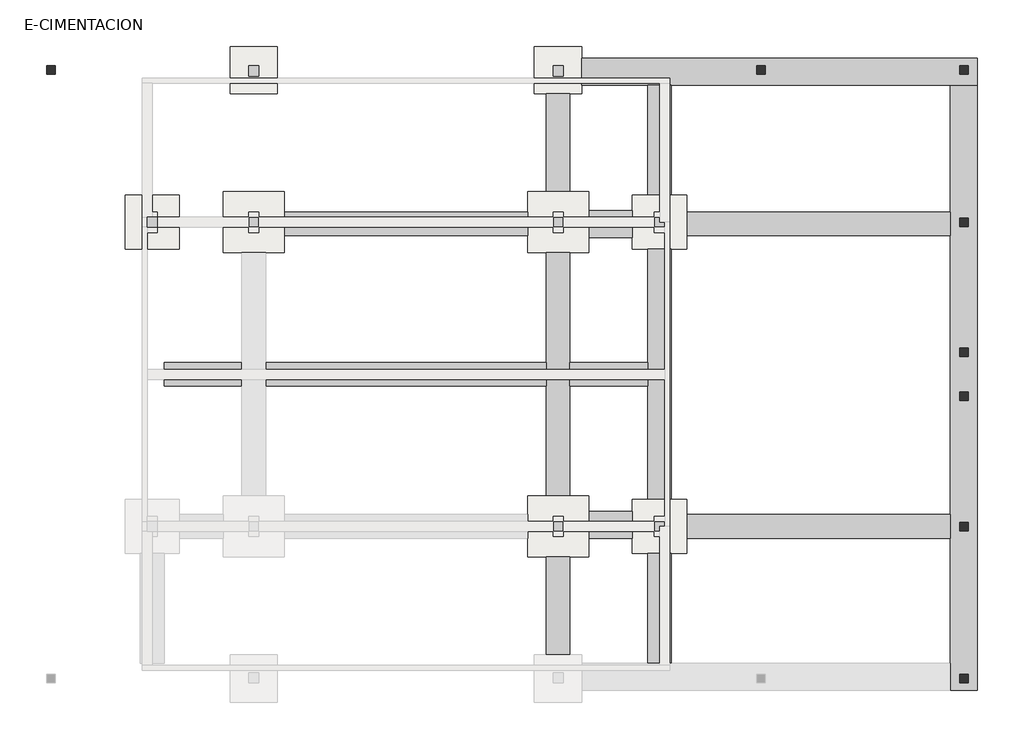
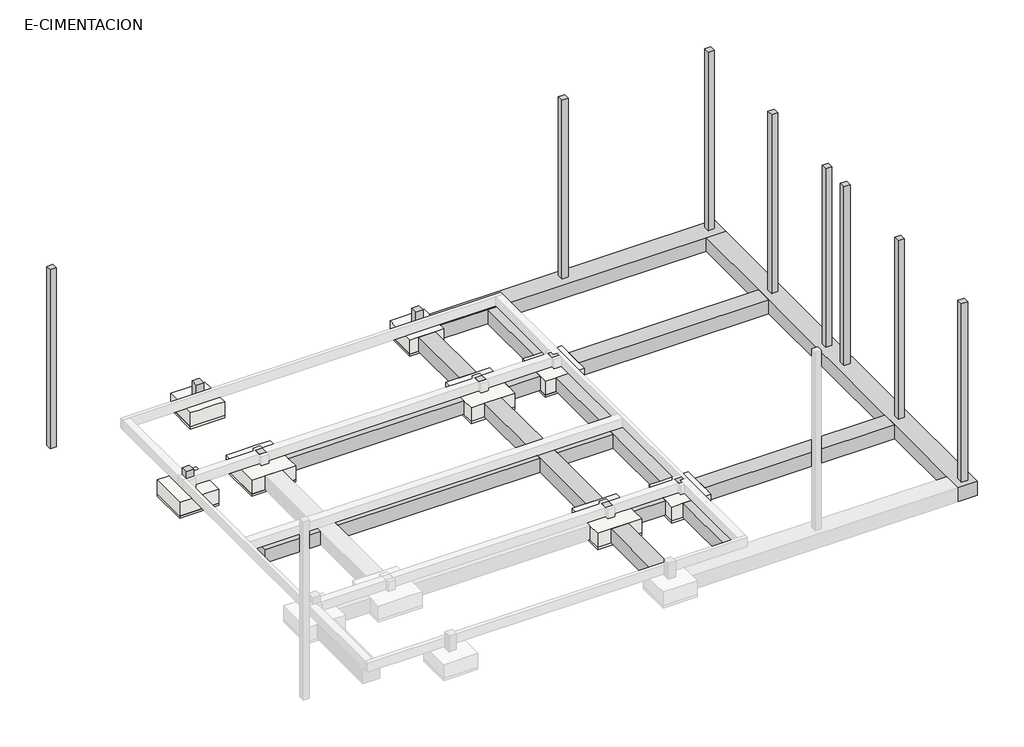
# One storey, part 2 of 2: 16 columns, 14 beams, 8 slabs.
"""IFC4 building model written with IfcOpenShell, lengths in millimetres."""

from ifc_helpers import new_model, si_unit, frame, origin, place, context, project, spatial, polyline, outline, extrude, faceted_brep, element, save

model = new_model("IFC4")

# Units and contexts
model_context = context("Model", 3, world=origin())
ifc_project = project(units=[si_unit("LENGTHUNIT", "METRE", prefix="MILLI")], contexts=[model_context])

# Site, building, storey
site = spatial("IfcSite", under=ifc_project)
building = spatial("IfcBuilding", under=site)
storey = spatial("IfcBuildingStorey", under=building, Name="E-CIMENTACION", Elevation=-900.0)

# Beams
placement = place(None, origin())
element("IfcBeam", 1, ObjectType="E-VIGA-Hormigon : E-VIGA-Hormigon", at=placement, inside=storey, context=model_context, shape_type="SweptSolid", body=[
    extrude(outline(polyline([(-12350.0, -700.0), (-11650.0, -700.0), (-11650.0, -3600.0), (-12350.0, -3600.0), (-12350.0, -700.0)])), frame((0.0, 0.0, -1500.0), z_axis=(0.0, 0.0, 1.0), x_axis=(1.0, 0.0, 0.0)), (0.0, 0.0, 1.0), 600.0),
])
element("IfcBeam", 2, ObjectType="E-VIGA-Hormigon : E-VIGA-Hormigon", at=placement, inside=storey, context=model_context, shape_type="Brep", body=[
    faceted_brep([(-12350.0, -5400.0, -900.0), (-12350.0, -5400.0, -1500.0), (-12350.0, -8650.0, -1500.0), (-12350.0, -9350.0, -1500.0), (-12350.0, -12600.0, -1500.0), (-12350.0, -12600.0, -900.0), (-12350.0, -9350.0, -900.0), (-12350.0, -8650.0, -900.0), (-11650.0, -5400.0, -1500.0), (-11650.0, -8650.0, -1500.0), (-11650.0, -9350.0, -1500.0), (-11650.0, -12600.0, -1500.0), (-11650.0, -5400.0, -900.0), (-11650.0, -8650.0, -900.0), (-11650.0, -9350.0, -900.0), (-11650.0, -12600.0, -900.0)], [[[0, 1, 2, 3, 4, 5, 6, 7]], [[1, 8, 9, 10, 11, 4, 3, 2]], [[8, 12, 13, 14, 15, 11, 10, 9]], [[12, 0, 7, 6, 5, 15, 14, 13]], [[1, 0, 12, 8]], [[5, 4, 11, 15]]]),
])
element("IfcBeam", 3, ObjectType="E-VIGA-Hormigon : E-VIGA-Hormigon", at=placement, inside=storey, context=model_context, shape_type="SweptSolid", body=[
    extrude(outline(polyline([(-11650.0, -17300.0), (-12350.0, -17300.0), (-12350.0, -14400.0), (-11650.0, -14400.0), (-11650.0, -17300.0)])), frame((0.0, 0.0, -1500.0), z_axis=(0.0, 0.0, 1.0), x_axis=(1.0, 0.0, 0.0)), (0.0, 0.0, 1.0), 600.0),
])
element("IfcBeam", 4, ObjectType="E-VIGA-Hormigon : E-VIGA-Hormigon", at=placement, inside=storey, context=model_context, shape_type="Brep", body=[
    faceted_brep([(400.0, -450.0, -1500.0), (400.0, -450.0, -900.0), (-400.0, -450.0, -900.0), (-8650.0, -450.0, -900.0), (-9350.0, -450.0, -900.0), (-11300.0, -450.0, -900.0), (-11300.0, -450.0, -1500.0), (-9350.0, -450.0, -1500.0), (-8650.0, -450.0, -1500.0), (-400.0, -450.0, -1500.0), (400.0, 350.0, -1500.0), (-11300.0, 350.0, -1500.0), (400.0, 350.0, -900.0), (-11300.0, 350.0, -900.0)], [[[0, 1, 2, 3, 4, 5, 6, 7, 8, 9]], [[10, 0, 9, 8, 7, 6, 11]], [[12, 10, 11, 13]], [[1, 12, 13, 5, 4, 3, 2]], [[6, 5, 13, 11]], [[1, 0, 10, 12]]]),
])
element("IfcBeam", 5, ObjectType="E-VIGA-Hormigon : E-VIGA-Hormigon", at=placement, inside=storey, context=model_context, shape_type="Brep", body=[
    faceted_brep([(-400.0, -18350.0, -1500.0), (-400.0, -18350.0, -900.0), (-400.0, -17550.0, -900.0), (-400.0, -13850.0, -900.0), (-400.0, -13150.0, -900.0), (-400.0, -4900.0, -900.0), (-400.0, -4200.0, -900.0), (-400.0, -450.0, -900.0), (-400.0, -450.0, -1500.0), (-400.0, -4200.0, -1500.0), (-400.0, -4900.0, -1500.0), (-400.0, -13150.0, -1500.0), (-400.0, -13850.0, -1500.0), (-400.0, -17550.0, -1500.0), (400.0, -18350.0, -1500.0), (400.0, -450.0, -1500.0), (400.0, -18350.0, -900.0), (400.0, -450.0, -900.0)], [[[0, 1, 2, 3, 4, 5, 6, 7, 8, 9, 10, 11, 12, 13]], [[14, 0, 13, 12, 11, 10, 9, 8, 15]], [[16, 14, 15, 17]], [[1, 16, 17, 7, 6, 5, 4, 3, 2]], [[8, 7, 17, 15]], [[1, 0, 14, 16]]]),
])
element("IfcBeam", 6, ObjectType="E-VIGA-Hormigon : E-VIGA-Hormigon", at=placement, inside=storey, context=model_context, shape_type="SweptSolid", body=[
    extrude(outline(polyline([(-400.0, -4200.0), (-400.0, -4900.0), (-8200.0, -4900.0), (-8200.0, -4200.0), (-400.0, -4200.0)])), frame((0.0, 0.0, -1500.0), z_axis=(0.0, 0.0, 1.0), x_axis=(1.0, 0.0, 0.0)), (0.0, 0.0, 1.0), 600.0),
])
element("IfcBeam", 7, ObjectType="E-VIGA-Hormigon : E-VIGA-Hormigon", at=placement, inside=storey, context=model_context, shape_type="SweptSolid", body=[
    extrude(outline(polyline([(-400.0, -13150.0), (-400.0, -13850.0), (-8200.0, -13850.0), (-8200.0, -13150.0), (-400.0, -13150.0)])), frame((0.0, 0.0, -1500.0), z_axis=(0.0, 0.0, 1.0), x_axis=(1.0, 0.0, 0.0)), (0.0, 0.0, 1.0), 600.0),
])
element("IfcBeam", 8, ObjectType="E-VIGA-Hormigon : E-VIGA-Hormigon", at=placement, inside=storey, context=model_context, shape_type="SweptSolid", body=[
    extrude(outline(polyline([(-11100.0, -4950.0), (-11100.0, -4150.0), (-9800.0, -4150.0), (-9800.0, -4950.0), (-11100.0, -4950.0)])), frame((0.0, 0.0, -1500.0), z_axis=(0.0, 0.0, 1.0), x_axis=(1.0, 0.0, 0.0)), (0.0, 0.0, 1.0), 600.0),
])
element("IfcBeam", 9, ObjectType="E-VIGA-Hormigon : E-VIGA-Hormigon", at=placement, inside=storey, context=model_context, shape_type="SweptSolid", body=[
    extrude(outline(polyline([(-11100.0, -13850.0), (-11100.0, -13050.0), (-9800.0, -13050.0), (-9800.0, -13850.0), (-11100.0, -13850.0)])), frame((0.0, 0.0, -1500.0), z_axis=(0.0, 0.0, 1.0), x_axis=(1.0, 0.0, 0.0)), (0.0, 0.0, 1.0), 600.0),
])
element("IfcBeam", 10, ObjectType="E-VIGA-Hormigon : E-VIGA-Hormigon", at=placement, inside=storey, context=model_context, shape_type="SweptSolid", body=[
    extrude(outline(polyline([(-20100.0, -4900.0), (-20100.0, -4200.0), (-12900.0, -4200.0), (-12900.0, -4900.0), (-20100.0, -4900.0)])), frame((0.0, 0.0, -1500.0), z_axis=(0.0, 0.0, 1.0), x_axis=(1.0, 0.0, 0.0)), (0.0, 0.0, 1.0), 600.0),
])
element("IfcBeam", 11, ObjectType="E-VIGA-Hormigon : E-VIGA-Hormigon", at=placement, inside=storey, context=model_context, shape_type="Brep", body=[
    faceted_brep([(-9350.0, -5300.0, -900.0), (-9350.0, -5300.0, -1500.0), (-9350.0, -8650.0, -1500.0), (-9350.0, -9350.0, -1500.0), (-9350.0, -12700.0, -1500.0), (-9350.0, -12700.0, -900.0), (-9350.0, -9350.0, -900.0), (-9350.0, -8650.0, -900.0), (-8650.0, -5300.0, -1500.0), (-8650.0, -12700.0, -1500.0), (-8650.0, -5300.0, -900.0), (-8650.0, -12700.0, -900.0)], [[[0, 1, 2, 3, 4, 5, 6, 7]], [[1, 8, 9, 4, 3, 2]], [[8, 10, 11, 9]], [[10, 0, 7, 6, 5, 11]], [[1, 0, 10, 8]], [[5, 4, 9, 11]]]),
])
element("IfcBeam", 12, ObjectType="E-VIGA-Hormigon : E-VIGA-Hormigon", at=placement, inside=storey, context=model_context, shape_type="SweptSolid", body=[
    extrude(outline(polyline([(-9350.0, -450.0), (-8650.0, -450.0), (-8650.0, -3700.0), (-9350.0, -3700.0), (-9350.0, -450.0)])), frame((0.0, 0.0, -1500.0), z_axis=(0.0, 0.0, 1.0), x_axis=(1.0, 0.0, 0.0)), (0.0, 0.0, 1.0), 600.0),
])
element("IfcBeam", 13, ObjectType="E-VIGA-Hormigon : E-VIGA-Hormigon", at=placement, inside=storey, context=model_context, shape_type="SweptSolid", body=[
    extrude(outline(polyline([(-8650.0, -17550.0), (-9350.0, -17550.0), (-9350.0, -14300.0), (-8650.0, -14300.0), (-8650.0, -17550.0)])), frame((0.0, 0.0, -1500.0), z_axis=(0.0, 0.0, 1.0), x_axis=(1.0, 0.0, 0.0)), (0.0, 0.0, 1.0), 600.0),
])
element("IfcBeam", 14, ObjectType="E-VIGA-Hormigon : E-VIGA-Hormigon", at=placement, inside=storey, context=model_context, shape_type="SweptSolid", body=[
    extrude(outline(polyline([(-9350.0, -8650.0), (-9350.0, -9350.0), (-11650.0, -9350.0), (-11650.0, -8650.0), (-9350.0, -8650.0)])), frame((0.0, 0.0, -1500.0), z_axis=(0.0, 0.0, 1.0), x_axis=(1.0, 0.0, 0.0)), (0.0, 0.0, 1.0), 600.0),
    extrude(outline(polyline([(-23650.0, -9350.0), (-23650.0, -8650.0), (-21350.0, -8650.0), (-21350.0, -9350.0), (-23650.0, -9350.0)])), frame((0.0, 0.0, -1500.0), z_axis=(0.0, 0.0, 1.0), x_axis=(1.0, 0.0, 0.0)), (0.0, 0.0, 1.0), 600.0),
    extrude(outline(polyline([(-12350.0, -8650.0), (-12350.0, -9350.0), (-20650.0, -9350.0), (-20650.0, -8650.0), (-12350.0, -8650.0)])), frame((0.0, 0.0, -1500.0), z_axis=(0.0, 0.0, 1.0), x_axis=(1.0, 0.0, 0.0)), (0.0, 0.0, 1.0), 600.0),
])

# Columns
element("IfcColumn", 15, ObjectType="Hormigón-Cuadrado-Pilar : PILAR 25X25", at=placement, inside=storey, context=model_context, shape_type="SweptSolid", body=[
    extrude(outline(polyline([(-26875.0, 125.0), (-26875.0, -125.0), (-27125.0, -125.0), (-27125.0, 125.0), (-26875.0, 125.0)])), frame((0.0, 0.0, -900.0), z_axis=(0.0, 0.0, 1.0), x_axis=(1.0, 0.0, 0.0)), (0.0, 0.0, 1.0), 7750.0),
])
element("IfcColumn", 16, ObjectType="Hormigón-Cuadrado-Pilar : PILAR 25X25", at=placement, inside=storey, context=model_context, shape_type="SweptSolid", body=[
    extrude(outline(polyline([(125.0, 125.0), (125.0, -125.0), (-125.0, -125.0), (-125.0, 125.0), (125.0, 125.0)])), frame((0.0, 0.0, -900.0), z_axis=(0.0, 0.0, 1.0), x_axis=(1.0, 0.0, 0.0)), (0.0, 0.0, 1.0), 7750.0),
])
element("IfcColumn", 17, ObjectType="Hormigón-Cuadrado-Pilar : PILAR 25X25", at=placement, inside=storey, context=model_context, shape_type="SweptSolid", body=[
    extrude(outline(polyline([(125.0, -4375.0), (125.0, -4625.0), (-125.0, -4625.0), (-125.0, -4375.0), (125.0, -4375.0)])), frame((0.0, 0.0, -900.0), z_axis=(0.0, 0.0, 1.0), x_axis=(1.0, 0.0, 0.0)), (0.0, 0.0, 1.0), 7750.0),
])
element("IfcColumn", 18, ObjectType="Hormigón-Cuadrado-Pilar : PILAR 25X25", at=placement, inside=storey, context=model_context, shape_type="Brep", body=[
    faceted_brep([(125.0, -8225.0, -900.0), (125.0, -8475.0, -900.0), (-125.0, -8475.0, -900.0), (-125.0, -8225.0, -900.0), (125.0, -8225.0, 6850.0), (125.0, -8475.0, 6850.0), (125.0, -8225.0, 2480.0), (125.0, -8225.0, 2730.0), (125.0, -8225.0, 6600.0), (-125.0, -8475.0, 6850.0), (-125.0, -8225.0, 6850.0), (-125.0, -8225.0, 6600.0), (-125.0, -8225.0, 2730.0), (-125.0, -8225.0, 2480.0)], [[[0, 1, 2, 3]], [[4, 5, 1, 0, 6, 7, 8]], [[5, 9, 2, 1]], [[9, 10, 11, 12, 13, 3, 2]], [[10, 4, 8, 7, 6, 0, 3, 13, 12, 11]], [[4, 10, 9, 5]]]),
])
element("IfcColumn", 19, ObjectType="Hormigón-Cuadrado-Pilar : PILAR 25X25", at=placement, inside=storey, context=model_context, shape_type="SweptSolid", body=[
    extrude(outline(polyline([(125.0, -13375.0), (125.0, -13625.0), (-125.0, -13625.0), (-125.0, -13375.0), (125.0, -13375.0)])), frame((0.0, 0.0, -900.0), z_axis=(0.0, 0.0, 1.0), x_axis=(1.0, 0.0, 0.0)), (0.0, 0.0, 1.0), 7750.0),
])
element("IfcColumn", 20, ObjectType="Hormigón-Cuadrado-Pilar : PILAR 25X25", at=placement, inside=storey, context=model_context, shape_type="SweptSolid", body=[
    extrude(outline(polyline([(125.0, -17875.0), (125.0, -18125.0), (-125.0, -18125.0), (-125.0, -17875.0), (125.0, -17875.0)])), frame((0.0, 0.0, -900.0), z_axis=(0.0, 0.0, 1.0), x_axis=(1.0, 0.0, 0.0)), (0.0, 0.0, 1.0), 7750.0),
])
element("IfcColumn", 21, ObjectType="Hormigón-Cuadrado-Pilar : PILAR 25X25", at=placement, inside=storey, context=model_context, shape_type="SweptSolid", body=[
    extrude(outline(polyline([(-5875.0, 125.0), (-5875.0, -125.0), (-6125.0, -125.0), (-6125.0, 125.0), (-5875.0, 125.0)])), frame((0.0, 0.0, -900.0), z_axis=(0.0, 0.0, 1.0), x_axis=(1.0, 0.0, 0.0)), (0.0, 0.0, 1.0), 7750.0),
])
element("IfcColumn", 22, ObjectType="Hormigón-Cuadrado-Pilar : PILAR 25X25", at=placement, inside=storey, context=model_context, shape_type="Brep", body=[
    faceted_brep([(125.0, -9775.0, -900.0), (-125.0, -9775.0, -900.0), (-125.0, -9525.0, -900.0), (125.0, -9525.0, -900.0), (125.0, -9775.0, 6850.0), (125.0, -9775.0, 6600.0), (125.0, -9775.0, 2730.0), (125.0, -9775.0, 2480.0), (125.0, -9525.0, 6850.0), (-125.0, -9525.0, 6850.0), (-125.0, -9775.0, 2480.0), (-125.0, -9775.0, 2730.0), (-125.0, -9775.0, 6600.0), (-125.0, -9775.0, 6850.0)], [[[0, 1, 2, 3]], [[4, 5, 6, 7, 0, 3, 8]], [[8, 3, 2, 9]], [[9, 2, 1, 10, 11, 12, 13]], [[13, 12, 11, 10, 1, 0, 7, 6, 5, 4]], [[4, 8, 9, 13]]]),
])
element("IfcColumn", 23, ObjectType="Hormigón-Cuadrado-Pilar : PILAR 30X30", at=placement, inside=storey, context=model_context, shape_type="SweptSolid", body=[
    extrude(outline(polyline([(-20850.0, 125.0), (-20850.0, -175.0), (-21150.0, -175.0), (-21150.0, 125.0), (-20850.0, 125.0)])), frame((0.0, 0.0, -900.0), z_axis=(0.0, 0.0, 1.0), x_axis=(1.0, 0.0, 0.0)), (0.0, 0.0, 1.0), 700.0),
])
element("IfcColumn", 24, ObjectType="Hormigón-Cuadrado-Pilar : PILAR 30X30", at=placement, inside=storey, context=model_context, shape_type="SweptSolid", body=[
    extrude(outline(polyline([(-11850.0, 125.0), (-11850.0, -175.0), (-12150.0, -175.0), (-12150.0, 125.0), (-11850.0, 125.0)])), frame((0.0, 0.0, -900.0), z_axis=(0.0, 0.0, 1.0), x_axis=(1.0, 0.0, 0.0)), (0.0, 0.0, 1.0), 700.0),
])
element("IfcColumn", 25, ObjectType="Hormigón-Cuadrado-Pilar : PILAR 30X30", at=placement, inside=storey, context=model_context, shape_type="SweptSolid", body=[
    extrude(outline(polyline([(-20850.0, -4350.0), (-20850.0, -4650.0), (-21150.0, -4650.0), (-21150.0, -4350.0), (-20850.0, -4350.0)])), frame((0.0, 0.0, -900.0), z_axis=(0.0, 0.0, 1.0), x_axis=(1.0, 0.0, 0.0)), (0.0, 0.0, 1.0), 400.0),
])
element("IfcColumn", 26, ObjectType="Hormigón-Cuadrado-Pilar : PILAR 30X30", at=placement, inside=storey, context=model_context, shape_type="SweptSolid", body=[
    extrude(outline(polyline([(-11850.0, -13350.0), (-11850.0, -13650.0), (-12150.0, -13650.0), (-12150.0, -13350.0), (-11850.0, -13350.0)])), frame((0.0, 0.0, -900.0), z_axis=(0.0, 0.0, 1.0), x_axis=(1.0, 0.0, 0.0)), (0.0, 0.0, 1.0), 400.0),
])
element("IfcColumn", 27, ObjectType="Hormigón-Cuadrado-Pilar : PILAR 30X30", at=placement, inside=storey, context=model_context, shape_type="SweptSolid", body=[
    extrude(outline(polyline([(-11850.0, -4350.0), (-11850.0, -4650.0), (-12150.0, -4650.0), (-12150.0, -4350.0), (-11850.0, -4350.0)])), frame((0.0, 0.0, -900.0), z_axis=(0.0, 0.0, 1.0), x_axis=(1.0, 0.0, 0.0)), (0.0, 0.0, 1.0), 400.0),
])
element("IfcColumn", 28, ObjectType="Hormigón-Cuadrado-Pilar : PILAR 30X30", at=placement, inside=storey, context=model_context, shape_type="SweptSolid", body=[
    extrude(outline(polyline([(-23850.0, -4350.0), (-23850.0, -4650.0), (-24150.0, -4650.0), (-24150.0, -4350.0), (-23850.0, -4350.0)])), frame((0.0, 0.0, -500.0), z_axis=(0.0, 0.0, 1.0), x_axis=(1.0, 0.0, 0.0)), (0.0, 0.0, 1.0), 300.0),
])
element("IfcColumn", 29, ObjectType="Hormigón-Cuadrado-Pilar : PILAR 30X30", at=placement, inside=storey, context=model_context, shape_type="SweptSolid", body=[
    extrude(outline(polyline([(-9150.0, -13650.0), (-9150.0, -13350.0), (-8850.0, -13350.0), (-8850.0, -13500.0), (-9000.0, -13500.0), (-9000.0, -13650.0), (-9150.0, -13650.0)])), frame((0.0, 0.0, -900.0), z_axis=(0.0, 0.0, 1.0), x_axis=(1.0, 0.0, 0.0)), (0.0, 0.0, 1.0), 400.0),
])
element("IfcColumn", 30, ObjectType="Hormigón-Cuadrado-Pilar : PILAR 30X30", at=placement, inside=storey, context=model_context, shape_type="SweptSolid", body=[
    extrude(outline(polyline([(-8850.0, -4650.0), (-9150.0, -4650.0), (-9150.0, -4350.0), (-9000.0, -4350.0), (-9000.0, -4500.0), (-8850.0, -4500.0), (-8850.0, -4650.0)])), frame((0.0, 0.0, -900.0), z_axis=(0.0, 0.0, 1.0), x_axis=(1.0, 0.0, 0.0)), (0.0, 0.0, 1.0), 400.0),
])

# Slabs
element("IfcSlab", 31, ObjectType="E-ZAPATA : E-ZAPATA", at=placement, inside=storey, context=model_context, shape_type="SolidModel", body=[
    faceted_brep([(-12700.0, 700.0, -900.0), (-12700.0, 350.0, -900.0), (-12700.0, -450.0, -900.0), (-12700.0, -700.0, -900.0), (-12350.0, -700.0, -900.0), (-11650.0, -700.0, -900.0), (-11300.0, -700.0, -900.0), (-11300.0, -450.0, -900.0), (-11300.0, 350.0, -900.0), (-11300.0, 700.0, -900.0), (-12700.0, 700.0, -1500.0), (-11300.0, 700.0, -1500.0), (-11300.0, 350.0, -1500.0), (-11300.0, -450.0, -1500.0), (-11300.0, -700.0, -1500.0), (-11650.0, -700.0, -1500.0), (-12350.0, -700.0, -1500.0), (-12700.0, -700.0, -1500.0), (-12700.0, -450.0, -1500.0), (-12700.0, 350.0, -1500.0)], [[[0, 1, 2, 3, 4, 5, 6, 7, 8, 9]], [[10, 11, 12, 13, 14, 15, 16, 17, 18, 19]], [[0, 9, 11, 10]], [[9, 8, 7, 6, 14, 13, 12, 11]], [[6, 5, 4, 3, 17, 16, 15, 14]], [[3, 2, 1, 0, 10, 19, 18, 17]]]),
    extrude(outline(polyline([(-11300.0, 700.0), (-11300.0, -700.0), (-12700.0, -700.0), (-12700.0, 700.0), (-11300.0, 700.0)])), frame((0.0, 0.0, -1600.0), z_axis=(0.0, 0.0, 1.0), x_axis=(1.0, 0.0, 0.0)), (0.0, 0.0, 1.0), 100.0),
])
element("IfcSlab", 32, ObjectType="E-ZAPATA : E-ZAPATA", at=placement, inside=storey, context=model_context, shape_type="SolidModel", body=[
    faceted_brep([(-21900.0, -3600.0, -900.0), (-21900.0, -4150.0, -900.0), (-21900.0, -4950.0, -900.0), (-21900.0, -5400.0, -900.0), (-21350.0, -5400.0, -900.0), (-20650.0, -5400.0, -900.0), (-20100.0, -5400.0, -900.0), (-20100.0, -4900.0, -900.0), (-20100.0, -4200.0, -900.0), (-20100.0, -3600.0, -900.0), (-20650.0, -3600.0, -900.0), (-21350.0, -3600.0, -900.0), (-21900.0, -3600.0, -1500.0), (-21350.0, -3600.0, -1500.0), (-20650.0, -3600.0, -1500.0), (-20100.0, -3600.0, -1500.0), (-20100.0, -4200.0, -1500.0), (-20100.0, -4900.0, -1500.0), (-20100.0, -5400.0, -1500.0), (-20650.0, -5400.0, -1500.0), (-21350.0, -5400.0, -1500.0), (-21900.0, -5400.0, -1500.0), (-21900.0, -4950.0, -1500.0), (-21900.0, -4150.0, -1500.0)], [[[0, 1, 2, 3, 4, 5, 6, 7, 8, 9, 10, 11]], [[12, 13, 14, 15, 16, 17, 18, 19, 20, 21, 22, 23]], [[0, 11, 10, 9, 15, 14, 13, 12]], [[9, 8, 7, 6, 18, 17, 16, 15]], [[6, 5, 4, 3, 21, 20, 19, 18]], [[3, 2, 1, 0, 12, 23, 22, 21]]]),
    extrude(outline(polyline([(-20100.0, -3600.0), (-20100.0, -5400.0), (-21900.0, -5400.0), (-21900.0, -3600.0), (-20100.0, -3600.0)])), frame((0.0, 0.0, -1600.0), z_axis=(0.0, 0.0, 1.0), x_axis=(1.0, 0.0, 0.0)), (0.0, 0.0, 1.0), 100.0),
])
element("IfcSlab", 33, ObjectType="E-ZAPATA : E-ZAPATA", at=placement, inside=storey, context=model_context, shape_type="SolidModel", body=[
    faceted_brep([(-12900.0, -3600.0, -900.0), (-12900.0, -4200.0, -900.0), (-12900.0, -4900.0, -900.0), (-12900.0, -5400.0, -900.0), (-12350.0, -5400.0, -900.0), (-11650.0, -5400.0, -900.0), (-11100.0, -5400.0, -900.0), (-11100.0, -4950.0, -900.0), (-11100.0, -4150.0, -900.0), (-11100.0, -3600.0, -900.0), (-11650.0, -3600.0, -900.0), (-12350.0, -3600.0, -900.0), (-12900.0, -3600.0, -1500.0), (-12350.0, -3600.0, -1500.0), (-11650.0, -3600.0, -1500.0), (-11100.0, -3600.0, -1500.0), (-11100.0, -4150.0, -1500.0), (-11100.0, -4950.0, -1500.0), (-11100.0, -5400.0, -1500.0), (-11650.0, -5400.0, -1500.0), (-12350.0, -5400.0, -1500.0), (-12900.0, -5400.0, -1500.0), (-12900.0, -4900.0, -1500.0), (-12900.0, -4200.0, -1500.0)], [[[0, 1, 2, 3, 4, 5, 6, 7, 8, 9, 10, 11]], [[12, 13, 14, 15, 16, 17, 18, 19, 20, 21, 22, 23]], [[0, 11, 10, 9, 15, 14, 13, 12]], [[9, 8, 7, 6, 18, 17, 16, 15]], [[6, 5, 4, 3, 21, 20, 19, 18]], [[3, 2, 1, 0, 12, 23, 22, 21]]]),
    extrude(outline(polyline([(-11100.0, -3600.0), (-11100.0, -5400.0), (-12900.0, -5400.0), (-12900.0, -3600.0), (-11100.0, -3600.0)])), frame((0.0, 0.0, -1600.0), z_axis=(0.0, 0.0, 1.0), x_axis=(1.0, 0.0, 0.0)), (0.0, 0.0, 1.0), 100.0),
])
element("IfcSlab", 34, ObjectType="E-ZAPATA : E-ZAPATA", at=placement, inside=storey, context=model_context, shape_type="SolidModel", body=[
    faceted_brep([(-24800.0, -5300.0, -900.0), (-24350.0, -5300.0, -900.0), (-23650.0, -5300.0, -900.0), (-23200.0, -5300.0, -900.0), (-23200.0, -4950.0, -900.0), (-23200.0, -4150.0, -900.0), (-23200.0, -3700.0, -900.0), (-23650.0, -3700.0, -900.0), (-24350.0, -3700.0, -900.0), (-24800.0, -3700.0, -900.0), (-24800.0, -5300.0, -1500.0), (-24800.0, -3700.0, -1500.0), (-24350.0, -3700.0, -1500.0), (-23650.0, -3700.0, -1500.0), (-23200.0, -3700.0, -1500.0), (-23200.0, -4150.0, -1500.0), (-23200.0, -4950.0, -1500.0), (-23200.0, -5300.0, -1500.0), (-23650.0, -5300.0, -1500.0), (-24350.0, -5300.0, -1500.0)], [[[0, 1, 2, 3, 4, 5, 6, 7, 8, 9]], [[10, 11, 12, 13, 14, 15, 16, 17, 18, 19]], [[0, 9, 11, 10]], [[9, 8, 7, 6, 14, 13, 12, 11]], [[6, 5, 4, 3, 17, 16, 15, 14]], [[3, 2, 1, 0, 10, 19, 18, 17]]]),
    extrude(outline(polyline([(-24800.0, -3700.0), (-23200.0, -3700.0), (-23200.0, -5300.0), (-24800.0, -5300.0), (-24800.0, -3700.0)])), frame((0.0, 0.0, -1600.0), z_axis=(0.0, 0.0, 1.0), x_axis=(1.0, 0.0, 0.0)), (0.0, 0.0, 1.0), 100.0),
])
element("IfcSlab", 35, ObjectType="E-ZAPATA : E-ZAPATA", at=placement, inside=storey, context=model_context, shape_type="SolidModel", body=[
    faceted_brep([(-9800.0, -3700.0, -900.0), (-9800.0, -4150.0, -900.0), (-9800.0, -4950.0, -900.0), (-9800.0, -5300.0, -900.0), (-9350.0, -5300.0, -900.0), (-8650.0, -5300.0, -900.0), (-8200.0, -5300.0, -900.0), (-8200.0, -4900.0, -900.0), (-8200.0, -4200.0, -900.0), (-8200.0, -3700.0, -900.0), (-8650.0, -3700.0, -900.0), (-9350.0, -3700.0, -900.0), (-9800.0, -3700.0, -1500.0), (-9350.0, -3700.0, -1500.0), (-8650.0, -3700.0, -1500.0), (-8200.0, -3700.0, -1500.0), (-8200.0, -4200.0, -1500.0), (-8200.0, -4900.0, -1500.0), (-8200.0, -5300.0, -1500.0), (-8650.0, -5300.0, -1500.0), (-9350.0, -5300.0, -1500.0), (-9800.0, -5300.0, -1500.0), (-9800.0, -4950.0, -1500.0), (-9800.0, -4150.0, -1500.0)], [[[0, 1, 2, 3, 4, 5, 6, 7, 8, 9, 10, 11]], [[12, 13, 14, 15, 16, 17, 18, 19, 20, 21, 22, 23]], [[0, 11, 10, 9, 15, 14, 13, 12]], [[9, 8, 7, 6, 18, 17, 16, 15]], [[6, 5, 4, 3, 21, 20, 19, 18]], [[3, 2, 1, 0, 12, 23, 22, 21]]]),
    extrude(outline(polyline([(-8200.0, -3700.0), (-8200.0, -5300.0), (-9800.0, -5300.0), (-9800.0, -3700.0), (-8200.0, -3700.0)])), frame((0.0, 0.0, -1600.0), z_axis=(0.0, 0.0, 1.0), x_axis=(1.0, 0.0, 0.0)), (0.0, 0.0, 1.0), 100.0),
])
element("IfcSlab", 36, ObjectType="E-ZAPATA : E-ZAPATA", at=placement, inside=storey, context=model_context, shape_type="SolidModel", body=[
    faceted_brep([(-12900.0, -14400.0, -900.0), (-12350.0, -14400.0, -900.0), (-11650.0, -14400.0, -900.0), (-11100.0, -14400.0, -900.0), (-11100.0, -13850.0, -900.0), (-11100.0, -13050.0, -900.0), (-11100.0, -12600.0, -900.0), (-11650.0, -12600.0, -900.0), (-12350.0, -12600.0, -900.0), (-12900.0, -12600.0, -900.0), (-12900.0, -13150.0, -900.0), (-12900.0, -13850.0, -900.0), (-12900.0, -14400.0, -1500.0), (-12900.0, -13850.0, -1500.0), (-12900.0, -13150.0, -1500.0), (-12900.0, -12600.0, -1500.0), (-12350.0, -12600.0, -1500.0), (-11650.0, -12600.0, -1500.0), (-11100.0, -12600.0, -1500.0), (-11100.0, -13050.0, -1500.0), (-11100.0, -13850.0, -1500.0), (-11100.0, -14400.0, -1500.0), (-11650.0, -14400.0, -1500.0), (-12350.0, -14400.0, -1500.0)], [[[0, 1, 2, 3, 4, 5, 6, 7, 8, 9, 10, 11]], [[12, 13, 14, 15, 16, 17, 18, 19, 20, 21, 22, 23]], [[0, 12, 23, 22, 21, 3, 2, 1]], [[3, 21, 20, 19, 18, 6, 5, 4]], [[6, 18, 17, 16, 15, 9, 8, 7]], [[9, 15, 14, 13, 12, 0, 11, 10]]]),
    extrude(outline(polyline([(-11100.0, -14400.0), (-12900.0, -14400.0), (-12900.0, -12600.0), (-11100.0, -12600.0), (-11100.0, -14400.0)])), frame((0.0, 0.0, -1600.0), z_axis=(0.0, 0.0, 1.0), x_axis=(1.0, 0.0, 0.0)), (0.0, 0.0, 1.0), 100.0),
])
element("IfcSlab", 37, ObjectType="E-ZAPATA : E-ZAPATA", at=placement, inside=storey, context=model_context, shape_type="SolidModel", body=[
    faceted_brep([(-9800.0, -14300.0, -900.0), (-9350.0, -14300.0, -900.0), (-8650.0, -14300.0, -900.0), (-8200.0, -14300.0, -900.0), (-8200.0, -13850.0, -900.0), (-8200.0, -13150.0, -900.0), (-8200.0, -12700.0, -900.0), (-8650.0, -12700.0, -900.0), (-9350.0, -12700.0, -900.0), (-9800.0, -12700.0, -900.0), (-9800.0, -13050.0, -900.0), (-9800.0, -13850.0, -900.0), (-9800.0, -14300.0, -1500.0), (-9800.0, -13850.0, -1500.0), (-9800.0, -13050.0, -1500.0), (-9800.0, -12700.0, -1500.0), (-9350.0, -12700.0, -1500.0), (-8650.0, -12700.0, -1500.0), (-8200.0, -12700.0, -1500.0), (-8200.0, -13150.0, -1500.0), (-8200.0, -13850.0, -1500.0), (-8200.0, -14300.0, -1500.0), (-8650.0, -14300.0, -1500.0), (-9350.0, -14300.0, -1500.0)], [[[0, 1, 2, 3, 4, 5, 6, 7, 8, 9, 10, 11]], [[12, 13, 14, 15, 16, 17, 18, 19, 20, 21, 22, 23]], [[0, 12, 23, 22, 21, 3, 2, 1]], [[3, 21, 20, 19, 18, 6, 5, 4]], [[6, 18, 17, 16, 15, 9, 8, 7]], [[9, 15, 14, 13, 12, 0, 11, 10]]]),
    extrude(outline(polyline([(-8200.0, -14300.0), (-9800.0, -14300.0), (-9800.0, -12700.0), (-8200.0, -12700.0), (-8200.0, -14300.0)])), frame((0.0, 0.0, -1600.0), z_axis=(0.0, 0.0, 1.0), x_axis=(1.0, 0.0, 0.0)), (0.0, 0.0, 1.0), 100.0),
])
element("IfcSlab", 38, ObjectType="E-ZAPATA : E-ZAPATA", at=placement, inside=storey, context=model_context, shape_type="SolidModel", body=[
    faceted_brep([(-21700.0, 700.0, -900.0), (-21700.0, 350.0, -900.0), (-21700.0, -450.0, -900.0), (-21700.0, -700.0, -900.0), (-21350.0, -700.0, -900.0), (-20650.0, -700.0, -900.0), (-20300.0, -700.0, -900.0), (-20300.0, -450.0, -900.0), (-20300.0, 350.0, -900.0), (-20300.0, 700.0, -900.0), (-21700.0, 700.0, -1500.0), (-20300.0, 700.0, -1500.0), (-20300.0, 350.0, -1500.0), (-20300.0, -450.0, -1500.0), (-20300.0, -700.0, -1500.0), (-20650.0, -700.0, -1500.0), (-21350.0, -700.0, -1500.0), (-21700.0, -700.0, -1500.0), (-21700.0, -450.0, -1500.0), (-21700.0, 350.0, -1500.0)], [[[0, 1, 2, 3, 4, 5, 6, 7, 8, 9]], [[10, 11, 12, 13, 14, 15, 16, 17, 18, 19]], [[0, 9, 11, 10]], [[9, 8, 7, 6, 14, 13, 12, 11]], [[6, 5, 4, 3, 17, 16, 15, 14]], [[3, 2, 1, 0, 10, 19, 18, 17]]]),
    extrude(outline(polyline([(-20300.0, 700.0), (-20300.0, -700.0), (-21700.0, -700.0), (-21700.0, 700.0), (-20300.0, 700.0)])), frame((0.0, 0.0, -1600.0), z_axis=(0.0, 0.0, 1.0), x_axis=(1.0, 0.0, 0.0)), (0.0, 0.0, 1.0), 100.0),
])

save(model, "model.ifc")

# Revit data of these elements
# Type "E-VIGA-Hormigon : E-VIGA-Hormigon"
#   Numeration [instance default] = ""
#   Length [instance default] = 3.000 m
#   AnchoViga [instance default] = 0.200 m
#   AltoViga [instance default] = 0.300 m
# Type "Hormigón-Cuadrado-Pilar : PILAR 25X25"
#   b = 0.250 m
#   Structural Material [instance default] = Hormigón - Hormigón moldeado in situ
# Type "Hormigón-Cuadrado-Pilar : PILAR 30X30"
#   b = 0.300 m
#   Structural Material [instance default] = Hormigón - Hormigón moldeado in situ
# Type "E-ZAPATA : E-ZAPATA"
#   y1 [instance default] = 0.500 m
#   x1 [instance default] = 0.500 m
#   GrosorHormigonLimpieza [instance default] = 0.100 m
#   Width [instance default] = 1.000 m
#   Length [instance default] = 1.000 m
#   Foundation Thickness [instance default] = 0.500 m
#   ColocacionEjeY [instance default] = no
#   ColocacionEjeX [instance default] = no
#   HormigonLimpieza = none
#   Structural Material = none
# Elements 1, 2, 3, 6, 7, 10, 11, 12, 13, 14 (IfcBeam, "E-VIGA-Hormigon : E-VIGA-Hormigon")
#   Comments = ""
#   Numeration = ""
#   AnchoViga = 0.700 m
#   AltoViga = 0.600 m
#   Phase Created = Nueva construcción
#   Materials on its faces: "Concrete, Cast-in-Place, Gray"
# Elements 4, 5, 9 (IfcBeam, "E-VIGA-Hormigon : E-VIGA-Hormigon")
#   Comments = ""
#   Numeration = ""
#   AnchoViga = 0.800 m
#   AltoViga = 0.600 m
#   Phase Created = Nueva construcción
#   Materials on its faces: "Concrete, Cast-in-Place, Gray"
# Element 8 (IfcBeam, "E-VIGA-Hormigon : E-VIGA-Hormigon")
#   Comments = ""
#   Numeration = ""
#   Length = 3.000 m
#   AnchoViga = 0.800 m
#   AltoViga = 0.600 m
#   Phase Created = Nueva construcción
#   Materials on its faces: "Concrete, Cast-in-Place, Gray"
# Elements 15, 16, 17, 18, 19, 20, 21, 22 (IfcColumn, "Hormigón-Cuadrado-Pilar : PILAR 25X25")
#   Comments = ""
#   Structural Material = Hormigón - Hormigón moldeado in situ
#   Phase Created = Nueva construcción
#   Materials on its faces: "Hormigón - Hormigón moldeado in situ"
# Elements 23, 24, 25, 26, 27, 28, 29, 30 (IfcColumn, "Hormigón-Cuadrado-Pilar : PILAR 30X30")
#   Comments = ""
#   Structural Material = Hormigón - Hormigón moldeado in situ
#   Phase Created = Nueva construcción
#   Materials on its faces: "Hormigón - Hormigón moldeado in situ"
# Elements 31, 38 (IfcSlab, "E-ZAPATA : E-ZAPATA")
#   Comments = ""
#   y1 = 0.700 m
#   x1 = 0.700 m
#   Length = 1.400 m
#   GrosorHormigonLimpieza = 0.100 m
#   Foundation Thickness = 0.600 m
#   Width = 1.400 m
#   ColocacionEjeY = no
#   ColocacionEjeX = no
#   Phase Created = Nueva construcción
# Elements 32, 33, 36 (IfcSlab, "E-ZAPATA : E-ZAPATA")
#   Comments = ""
#   y1 = 0.900 m
#   x1 = 0.900 m
#   Length = 1.800 m
#   GrosorHormigonLimpieza = 0.100 m
#   Foundation Thickness = 0.600 m
#   Width = 1.800 m
#   ColocacionEjeY = no
#   ColocacionEjeX = no
#   Phase Created = Nueva construcción
# Elements 34, 35, 37 (IfcSlab, "E-ZAPATA : E-ZAPATA")
#   Comments = ""
#   y1 = 0.800 m
#   x1 = 0.800 m
#   Length = 1.600 m
#   GrosorHormigonLimpieza = 0.100 m
#   Foundation Thickness = 0.600 m
#   Width = 1.600 m
#   ColocacionEjeY = no
#   ColocacionEjeX = no
#   Phase Created = Nueva construcción
# Materials
#   "Hormigón - Hormigón moldeado in situ": class "Hormigón", colour RGB 192 192 192, transparency 0, Cost = 0
#   "Concrete, Cast-in-Place, Gray": class "Concrete", colour RGB 129 132 118, transparency 0, Description = "Cast-in-place concrete", Cost = 0
